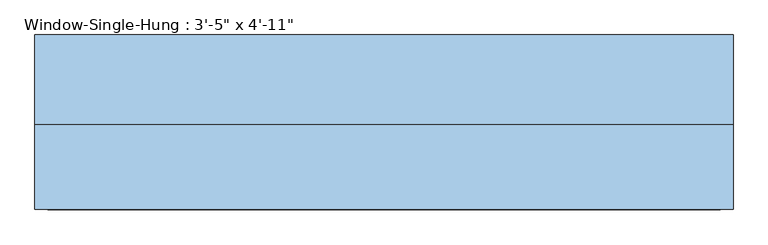
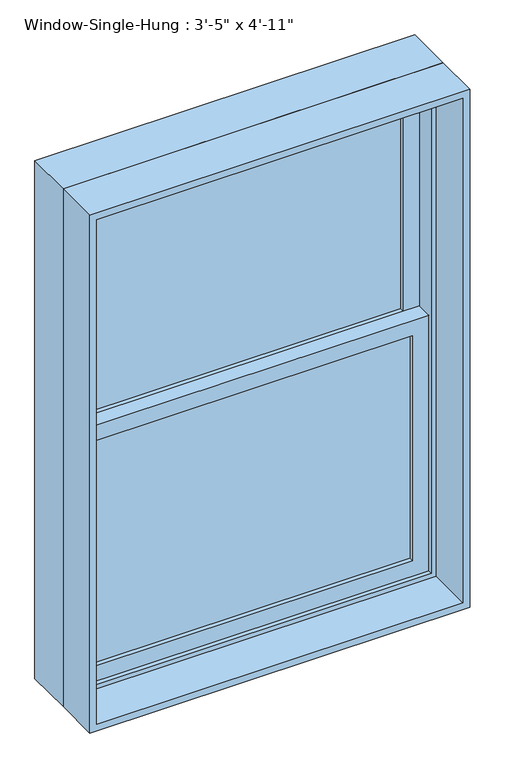
"""IFC4 building model written with IfcOpenShell, lengths in millimetres: window geometry."""

from ifc_helpers import new_model, si_unit, frame, origin, place, context, project, spatial, polyline, outline, extrude, source, transform, mapped, element, save


def window_84eda538(model_context):
    return source(origin(), model_context, "Body", "SweptSolid", [
        extrude(outline(polyline([(444.5, 50.8), (444.5, 44.45), (-444.5, 44.45), (-444.5, 50.8), (444.5, 50.8)])), frame((0.0, 0.0, 990.6), z_axis=(0.0, 0.0, 1.0), x_axis=(1.0, 0.0, 0.0)), (0.0, 0.0, 1.0), 650.875),
        extrude(outline(polyline([(-444.5, 38.1), (444.5, 38.1), (444.5, 31.75), (-444.5, 31.75), (-444.5, 38.1)])), frame((0.0, 0.0, 990.6), z_axis=(0.0, 0.0, 1.0), x_axis=(1.0, 0.0, 0.0)), (0.0, 0.0, 1.0), 650.875),
        extrude(outline(polyline([(444.5, 95.25), (444.5, 88.9), (-444.5, 88.9), (-444.5, 95.25), (444.5, 95.25)])), frame((0.0, 0.0, 1685.925), z_axis=(0.0, 0.0, 1.0), x_axis=(1.0, 0.0, 0.0)), (0.0, 0.0, 1.0), 650.875),
        extrude(outline(polyline([(-444.5, 82.55), (444.5, 82.55), (444.5, 76.2), (-444.5, 76.2), (-444.5, 82.55)])), frame((0.0, 0.0, 1685.925), z_axis=(0.0, 0.0, 1.0), x_axis=(1.0, 0.0, 0.0)), (0.0, 0.0, 1.0), 650.875),
        extrude(outline(polyline([(1685.925, -488.95), (946.15, -488.95), (946.15, 488.95), (1685.925, 488.95), (1685.925, -488.95)]), holes=[polyline([(1641.475, 444.5), (990.6, 444.5), (990.6, -444.5), (1641.475, -444.5), (1641.475, 444.5)])]), frame((0.0, 19.05, 0.0), z_axis=(0.0, 1.0, 0.0), x_axis=(0.0, 0.0, 1.0)), (0.0, 0.0, 1.0), 44.45),
        extrude(outline(polyline([(2381.25, -488.95), (1641.475, -488.95), (1641.475, 488.95), (2381.25, 488.95), (2381.25, -488.95)]), holes=[polyline([(2336.8, 444.5), (1685.925, 444.5), (1685.925, -444.5), (2336.8, -444.5), (2336.8, 444.5)])]), frame((0.0, 63.5, 0.0), z_axis=(0.0, 1.0, 0.0), x_axis=(0.0, 0.0, 1.0)), (0.0, 0.0, 1.0), 44.45),
        extrude(outline(polyline([(2413.0, -520.7), (914.4, -520.7), (914.4, 520.7), (2413.0, 520.7), (2413.0, -520.7)]), holes=[polyline([(2381.25, 488.95), (946.15, 488.95), (946.15, -488.95), (2381.25, -488.95), (2381.25, 488.95)])]), frame((0.0, 6.35, 0.0), z_axis=(0.0, 1.0, 0.0), x_axis=(0.0, 0.0, 1.0)), (0.0, 0.0, 1.0), 133.35),
        extrude(outline(polyline([(2413.0, 520.7), (2413.0, -520.7), (914.4, -520.7), (914.4, 520.7), (2413.0, 520.7)]), holes=[polyline([(2393.95, 501.65), (933.45, 501.65), (933.45, -501.65), (2393.95, -501.65), (2393.95, 501.65)])]), frame((0.0, -120.65, 0.0), z_axis=(0.0, 1.0, 0.0), x_axis=(0.0, 0.0, 1.0)), (0.0, 0.0, 1.0), 127.0),
    ])


if __name__ == "__main__":
    model = new_model("IFC4")
    model_context = context("Model", 3, world=origin())
    ifc_project = project(units=[si_unit("LENGTHUNIT", "METRE", prefix="MILLI")], contexts=[model_context])
    site = spatial("IfcSite", under=ifc_project)
    building = spatial("IfcBuilding", under=site)
    placement = place(None, origin())
    window_shape = window_84eda538(model_context)
    element("IfcWindow", 1, ObjectType="Window-Single-Hung : 3'-5\" x 4'-11\"", at=placement, inside=building, context=model_context, shape_type="MappedRepresentation", body=[
        mapped(window_shape, transform((0.0, 0.0, 0.0), x_axis=(1.0, 0.0, 0.0), y_axis=(0.0, 1.0, 0.0), z_axis=(0.0, 0.0, 1.0))),
    ])
    save(model, "model.ifc")

# Revit data of these elements
# Type "Window-Single-Hung : 3'-5\" x 4'-11\""
#   Type Mark = "03"
#   Fire Rating = "0.5h"
#   Construction Type Id = "DG-DR"
#   Assembly Code = "B2020100"
#   Analytic Construction = "Double glazing - domestic"
#   Wall Thickness [instance default] = 0' - 6"
#   Window Inset [instance default] = 0' - 0"
#   Visual Light Transmittance = 0.81
#   Thermal Resistance (R) = 0.319569 (m²·K)/W
#   Solar Heat Gain Coefficient = 0.76
#   Muntin Width = 2' - 11"
#   Muntin Height = 2' - 1 5/8"
#   Interior Wall Closure [instance default] = 0' - 1 1/2"
#   Rough Width = 3' - 5 1/2"
#   Rough Height = 4' - 11 1/2"
#   Frame Extension [instance default] = 0' - 1 1/4"
#   Exterior Wall Closure [instance default] = 0' - 0 1/2"
#   Extension Jamb [instance default] = 0' - 1 1/2"
#   Heat Transfer Coefficient (U) = 3.12929 W/(m²·K)
#   Height = 4' - 11"
#   Width = 3' - 5"
#   Top Muntin Visibility = no
#   Indicator Visibility = no
#   Extension Jamb Visibility [instance default] = yes
#   Interior Trim Visibility [instance default] = yes
#   Exterior Trim Visibility [instance default] = yes
#   Bottom Muntin Visibility = no
#   Muntin Pattern = Muntin Pattern_2x2 : Muntin Pattern_2x2
#   Interior Trim Material = 1X WOOD COMPOSITE TRIM
#   Interior Trim = Trim-Window-Interior-Flat : Picture Frame
#   Exterior Trim Material = 1X WOOD COMPOSITE TRIM
#   Exterior Trim = Trim-Window-Exterior-Flat : with Sill
#   Glass Panel Material = NEW DOUBLE HUNG WINDOWS (TYP.)
#   Exterior Frame Material = 1X WOOD COMPOSITE TRIM
#   Interior Frame Material = 1X WOOD COMPOSITE TRIM
#   Wall Closure = (empty or 0)
# Element 1 (IfcWindow, "Window-Single-Hung : 3'-5\" x 4'-11\"")
#   Wall Thickness = 0' - 9 1/2"
#   Extension Jamb = 0' - 5"
#   Materials on its faces: "1X WOOD COMPOSITE TRIM", "NEW DOUBLE HUNG WINDOWS (TYP.)"
# Materials
#   "1X WOOD COMPOSITE TRIM": class "Generic", colour RGB 88 61 61, transparency 0, Cost = 0
#   "NEW DOUBLE HUNG WINDOWS (TYP.)": class "Glass", colour RGB 218 227 224, transparency 0.85, Description = "Soda Lime Glass", Cost = 0
